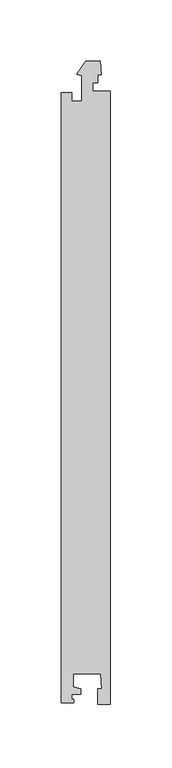
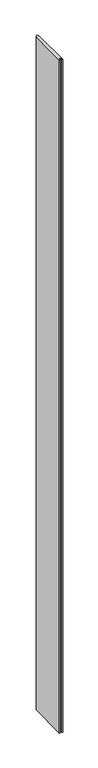
"""IFC4 building model written with IfcOpenShell, lengths in millimetres: proxy geometry, Generic Models 5:Generic Models 5:321804:Generic Models 5:321804 : Generic Models 5:Generic Models 5:321804:34 : Generic Models 5:Generic Models 5:321804:Generic Models 5:321804 : Generic Models 5:Generic Models 5:321804:300761."""

from ifc_helpers import new_model, si_unit, frame, origin, place, context, project, spatial, polyline, outline, extrude, source, transform, mapped, element, save


def generic_models_0761f36e(model_context):
    return source(origin(), model_context, "Body", "SweptSolid", [
        extrude(outline(polyline([(667625.2338797, -492410.833465), (667631.7338797, -492412.5751348), (667631.7338797, -492417.0251348), (667624.2338797, -492417.0251348), (667624.2338797, -492420.9751348), (667625.7338797, -492420.9751348), (667625.7338797, -492423.9751348), (667615.7338797, -492423.9751348), (667615.7338797, -491926.4751348), (667624.2338797, -491926.4751348), (667624.2338797, -491933.4251348), (667632.2338797, -491933.4251348), (667632.2338797, -491912.7091094), (667628.3059983, -491911.6566367), (667635.4133634, -491900.9751348), (667647.2715044, -491900.9751348), (667648.2338797, -491911.9751348), (667645.5338797, -491911.9751348), (667645.5338797, -491918.6001348), (667641.2338797, -491918.6001348), (667641.2338797, -491925.2251348), (667655.7338797, -491925.2251348), (667655.7338797, -492425.2251348), (667645.5338797, -492425.2251348), (667645.5338797, -492412.4751348), (667648.779534, -492412.4751348), (667647.72967, -492400.4751348), (667625.2338797, -492400.4751348), (667625.2338797, -492410.833465)])), frame((0.0, 0.0, -5.8417589), z_axis=(0.0, 0.0, 1.0), x_axis=(1.0, 0.0, 0.0)), (0.0, 0.0, 1.0), 8779.7126309),
    ])


if __name__ == "__main__":
    model = new_model("IFC4")
    model_context = context("Model", 3, world=origin())
    ifc_project = project(units=[si_unit("LENGTHUNIT", "METRE", prefix="MILLI")], contexts=[model_context])
    site = spatial("IfcSite", under=ifc_project)
    building = spatial("IfcBuilding", under=site)
    placement = place(None, origin())
    generic_models_shape = generic_models_0761f36e(model_context)
    element("IfcBuildingElementProxy", 1, Name="Generic Models 5:Generic Models 5:321804:Generic Models 5:321804 : Generic Models 5:Generic Models 5:321804:34 : Generic Models 5:Generic Models 5:321804:Generic Models 5:321804 : Generic Models 5:Generic Models 5:321804:300761", ObjectType="Generic Models 5:Generic Models 5:321804:Generic Models 5:321804 : Generic Models 5:Generic Models 5:321804:34 : Generic Models 5:Generic Models 5:321804:Generic Models 5:321804 : Generic Models 5:Generic Models 5:321804:300761", at=placement, inside=building, context=model_context, shape_type="MappedRepresentation", body=[
        mapped(generic_models_shape, transform((0.0, 0.0, 0.0), x_axis=(1.0, 0.0, 0.0), y_axis=(0.0, 1.0, 0.0), z_axis=(0.0, 0.0, 1.0))),
    ])
    save(model, "model.ifc")

# Revit data of these elements
# Type "Generic Models 5:Generic Models 5:321804:Generic Models 5:321804 : Generic Models 5:Generic Models 5:321804:34 : Generic Models 5:Generic Models 5:321804:Generic Models 5:321804 : Generic Models 5:Generic Models 5:321804:300761"
#   NameOverride = "Generic Models 5:Generic Models 5:321804:Generic Models 5:321804 : Generic Models 5:Generic Models 5:321804:300761"
#   ObjectTypeOverride = "Generic Models 5:321804 : Generic Models 5:Generic Models 5:321804"
#   Reference = "Generic Models 5"
#   Tag = "300761"
# Element 1 (IfcBuildingElementProxy, "Generic Models 5:Generic Models 5:321804:Generic Models 5:321804 : Generic Models 5:Generic Models 5:321804:34 : Generic Models 5:Generic Models 5:321804:Generic Models 5:321804 : Generic Models 5:Generic Models 5:321804:300761")
#   Materials on its faces: "POLYCARBONATE PANEL - ARCOPLUS 547"
# Materials
#   "POLYCARBONATE PANEL - ARCOPLUS 547": class "Unassigned", colour RGB 202 225 249, transparency 0.45, Cost = 0
